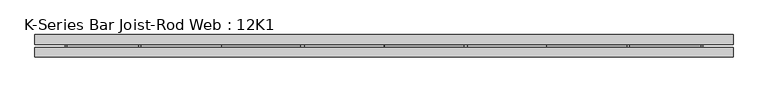
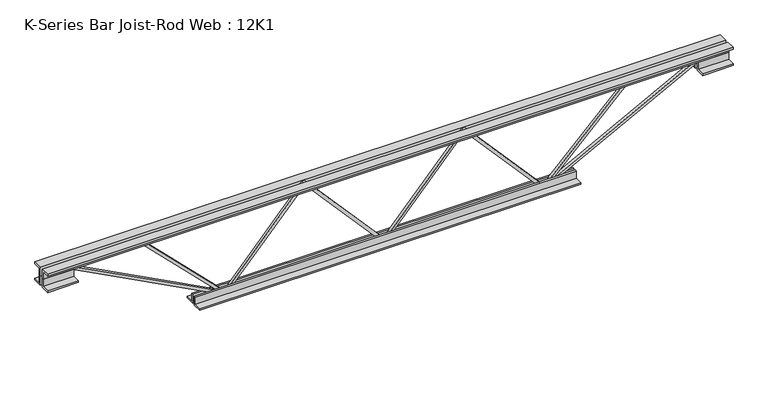
"""IFC4 building model written with IfcOpenShell, lengths in millimetres: beam geometry, K-Series Bar Joist-Rod Web : 12K1."""

from ifc_helpers import new_model, si_unit, frame, origin, place, context, project, spatial, polyline, outline, extrude, source, transform, mapped, element, save


def k_series_bar_joist_rod_web_12k1_28c7baf2(model_context):
    return source(origin(), model_context, "Body", "SweptSolid", [
        extrude(outline(polyline([(-141.2875, 0.0), (-150.8125, 0.0), (-150.8125, 5.3098219), (141.2875, 265.6598219), (141.2875, 267.7401781), (-150.8125, 528.0901781), (-150.8125, 533.4), (-141.2875, 533.4), (-141.2875, 532.3598219), (150.8125, 272.0098219), (150.8125, 261.3901781), (-141.2875, 1.0401781), (-141.2875, 0.0)])), frame((0.0, -4.7625, 0.0), z_axis=(0.0, 1.0, 0.0), x_axis=(0.0, 0.0, 1.0)), (0.0, 0.0, 1.0), 9.525),
        extrude(outline(polyline([(-141.2875, -533.4), (-150.8125, -533.4), (-150.8125, -528.0901781), (141.2875, -267.7401781), (141.2875, -265.6598219), (-150.8125, -5.3098219), (-150.8125, 0.0), (-141.2875, 0.0), (-141.2875, -1.0401781), (150.8125, -261.3901781), (150.8125, -272.0098219), (-141.2875, -532.3598219), (-141.2875, -533.4)])), frame((0.0, -4.7625, 0.0), z_axis=(0.0, 1.0, 0.0), x_axis=(0.0, 0.0, 1.0)), (0.0, 0.0, 1.0), 9.525),
        extrude(outline(polyline([(4.7625, 152.4), (36.5125, 152.4), (36.5125, 146.05), (11.1125, 146.05), (11.1125, 120.65), (4.7625, 120.65), (4.7625, 152.4)])), frame((-1143.0, 0.0, 0.0), z_axis=(1.0, 0.0, 0.0), x_axis=(0.0, 1.0, 0.0)), (0.0, 0.0, 1.0), 2286.0),
        extrude(outline(polyline([(-4.7625, 152.4), (-4.7625, 120.65), (-11.1125, 120.65), (-11.1125, 146.05), (-36.5125, 146.05), (-36.5125, 152.4), (-4.7625, 152.4)])), frame((-1143.0, 0.0, 0.0), z_axis=(1.0, 0.0, 0.0), x_axis=(0.0, 1.0, 0.0)), (0.0, 0.0, 1.0), 2286.0),
        extrude(outline(polyline([(-4.7625, 88.9), (-36.5125, 88.9), (-36.5125, 95.25), (-11.1125, 95.25), (-11.1125, 120.65), (-4.7625, 120.65), (-4.7625, 88.9)])), frame((-1143.0, 0.0, 0.0), z_axis=(1.0, 0.0, 0.0), x_axis=(0.0, 1.0, 0.0)), (0.0, 0.0, 1.0), 101.6),
        extrude(outline(polyline([(36.5125, 88.9), (4.7625, 88.9), (4.7625, 120.65), (11.1125, 120.65), (11.1125, 95.25), (36.5125, 95.25), (36.5125, 88.9)])), frame((-1143.0, 0.0, 0.0), z_axis=(1.0, 0.0, 0.0), x_axis=(0.0, 1.0, 0.0)), (0.0, 0.0, 1.0), 101.6),
        extrude(outline(polyline([(4.7625, 88.9), (4.7625, 120.65), (11.1125, 120.65), (11.1125, 95.25), (36.5125, 95.25), (36.5125, 88.9), (4.7625, 88.9)])), frame((1041.4, 0.0, 0.0), z_axis=(1.0, 0.0, 0.0), x_axis=(0.0, 1.0, 0.0)), (0.0, 0.0, 1.0), 101.6),
        extrude(outline(polyline([(-4.7625, 88.9), (-36.5125, 88.9), (-36.5125, 95.25), (-11.1125, 95.25), (-11.1125, 120.65), (-4.7625, 120.65), (-4.7625, 88.9)])), frame((1041.4, 0.0, 0.0), z_axis=(1.0, 0.0, 0.0), x_axis=(0.0, 1.0, 0.0)), (0.0, 0.0, 1.0), 101.6),
        extrude(outline(polyline([(4.7625, -152.4), (4.7625, -120.65), (11.1125, -120.65), (11.1125, -146.05), (36.5125, -146.05), (36.5125, -152.4), (4.7625, -152.4)])), frame((-635.0, 0.0, 0.0), z_axis=(1.0, 0.0, 0.0), x_axis=(0.0, 1.0, 0.0)), (0.0, 0.0, 1.0), 1270.0),
        extrude(outline(polyline([(-4.7625, -152.4), (-36.5125, -152.4), (-36.5125, -146.05), (-11.1125, -146.05), (-11.1125, -120.65), (-4.7625, -120.65), (-4.7625, -152.4)])), frame((-635.0, 0.0, 0.0), z_axis=(1.0, 0.0, 0.0), x_axis=(0.0, 1.0, 0.0)), (0.0, 0.0, 1.0), 1270.0),
        extrude(outline(polyline([(0.0, -9.525), (0.0, 0.0), (573.7533355, 0.0), (573.7533355, -9.525), (0.0, -9.525)])), frame((-1043.6137714, 4.7625, 116.4332925), z_axis=(0.4648338989895139, 0.0, 0.885397902838157), x_axis=(0.885397902838157, 0.0, -0.4648338989895139)), (0.0, 0.0, 1.0), 9.525),
        extrude(outline(polyline([(0.0, -9.525), (0.0, 0.0), (377.1707571, 0.0), (377.1707571, -9.525), (0.0, -9.525)])), frame((-803.467596, 4.7625, 117.282404), z_axis=(0.7071067811861826, 0.0, 0.7071067811869124), x_axis=(0.7071067811869124, 0.0, -0.7071067811861826)), (0.0, 0.0, 1.0), 9.525),
        extrude(outline(polyline([(0.0, -9.525), (0.0, 0.0), (573.7533355, 0.0), (573.7533355, -9.525), (0.0, -9.525)])), frame((1043.6137714, -4.7625, 116.4332925), z_axis=(-0.46483389898949523, 0.0, 0.8853979028381668), x_axis=(-0.8853979028381668, 0.0, -0.46483389898949523)), (0.0, 0.0, 1.0), 9.525),
        extrude(outline(polyline([(4.7625, 4.7624999), (4.7625, -4.7624999), (-4.7625, -4.7624999), (-4.7625, 4.7624999), (4.7625, 4.7624999)])), frame((533.4, 0.0, -146.05), z_axis=(0.7071067811869194, 0.0, 0.7071067811861756), x_axis=(0.0, -1.0, 0.0)), (0.0, 0.0, 1.0), 377.1707571),
    ])


if __name__ == "__main__":
    model = new_model("IFC4")
    model_context = context("Model", 3, world=origin())
    ifc_project = project(units=[si_unit("LENGTHUNIT", "METRE", prefix="MILLI")], contexts=[model_context])
    site = spatial("IfcSite", under=ifc_project)
    building = spatial("IfcBuilding", under=site)
    placement = place(None, origin())
    k_series_bar_joist_rod_web_12k1_shape = k_series_bar_joist_rod_web_12k1_28c7baf2(model_context)
    element("IfcBeam", 1, ObjectType="K-Series Bar Joist-Rod Web : 12K1", at=placement, inside=building, context=model_context, shape_type="MappedRepresentation", body=[
        mapped(k_series_bar_joist_rod_web_12k1_shape, transform((0.0, 0.0, 0.0), x_axis=(1.0, 0.0, 0.0), y_axis=(0.0, 1.0, 0.0), z_axis=(0.0, 0.0, 1.0))),
    ])
    save(model, "model.ifc")

# Revit data of these elements
# Type "K-Series Bar Joist-Rod Web : 12K1"
#   Assembly Code = "B1010350"
#   Wt = 5
#   Web Thickness = 0' - 0 3/8"
#   Start Offset [instance default] = 0' - 0"
#   Start Extension [instance default] = 0' - 0"
#   Seat Length = 0' - 4"
#   Seat Depth = 0' - 2 1/2"
#   PanelArrayLength [instance default] = 20' - 0"
#   Panel [instance default] = 2' - 0"
#   End Offset [instance default] = 0' - 0"
#   End Extension [instance default] = 0' - 0"
#   End Panel = 2' - 0"
#   Cord Leg = 0' - 1 1/4"
#   Chord Thickness = 0' - 0 1/4"
#   Length [instance default] = 24' - 0"
#   Depth = 1' - 0"
#   PanelArrayNum [instance default] = 10
#   Structural Material = none
# Element 1 (IfcBeam, "K-Series Bar Joist-Rod Web : 12K1")
#   PanelArrayLength = 3' - 6"
#   Panel = 1' - 9"
#   PanelArrayNum = 2
